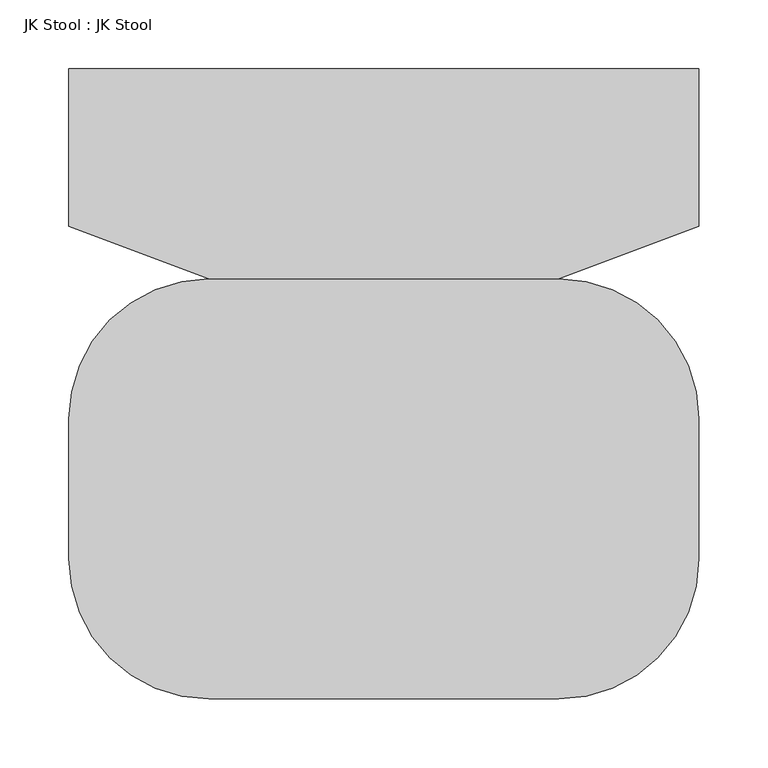
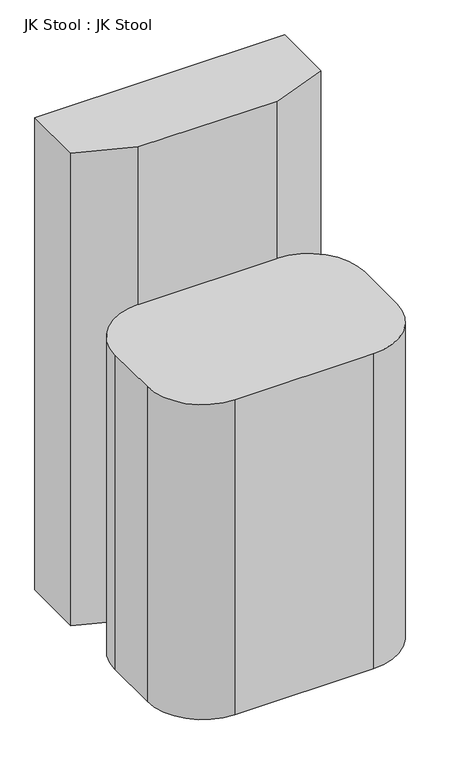
"""IFC4 building model written with IfcOpenShell, lengths in millimetres: furniture geometry, JK Stool : JK Stool."""

from ifc_helpers import new_model, si_unit, point, frame_2d, origin, origin_with_axes, place, context, project, spatial, polyline, circle_curve, trimmed, segment, composite_curve, outline, extrude, source, transform, mapped, element, save


def jk_stool_jk_stool_5b97b8dc(model_context):
    return source(origin(), model_context, "Body", "SweptSolid", [
        extrude(outline(polyline([(166.6573665, 262.1455296), (166.6573665, 147.8455296), (65.0573665, 109.7455296), (-188.9426335, 109.7455296), (-290.5426335, 147.8455296), (-290.5426335, 262.1455296), (166.6573665, 262.1455296)])), origin_with_axes(), (0.0, 0.0, 1.0), 914.4),
        extrude(outline(composite_curve([segment(trimmed(circle_curve(frame_2d((65.0573665, 8.1455296)), 101.6), [point((65.0573665, 109.7455296))], [point((166.6573665, 8.1455296))], False, "CARTESIAN"), True, "CONTINUOUS"), segment(polyline([(166.6573665, 8.1455296), (166.6573665, -93.4544704)]), True, "CONTINUOUS"), segment(trimmed(circle_curve(frame_2d((65.0573665, -93.4544704)), 101.6), [point((166.6573665, -93.4544704))], [point((65.0573665, -195.0544704))], False, "CARTESIAN"), True, "CONTINUOUS"), segment(polyline([(65.0573665, -195.0544704), (-188.9426335, -195.0544704)]), True, "CONTINUOUS"), segment(trimmed(circle_curve(frame_2d((-188.9426335, -93.4544704)), 101.6), [point((-188.9426335, -195.0544704))], [point((-290.5426335, -93.4544704))], False, "CARTESIAN"), True, "CONTINUOUS"), segment(polyline([(-290.5426335, -93.4544704), (-290.5426335, 8.1455296)]), True, "CONTINUOUS"), segment(trimmed(circle_curve(frame_2d((-188.9426335, 8.1455296)), 101.6), [point((-290.5426335, 8.1455296))], [point((-188.9426335, 109.7455296))], False, "CARTESIAN"), True, "CONTINUOUS"), segment(polyline([(-188.9426335, 109.7455296), (65.0573665, 109.7455296)]), True, "CONTINUOUS")], self_intersect=False)), origin_with_axes(), (0.0, 0.0, 1.0), 609.6),
    ])


if __name__ == "__main__":
    model = new_model("IFC4")
    model_context = context("Model", 3, world=origin())
    ifc_project = project(units=[si_unit("LENGTHUNIT", "METRE", prefix="MILLI")], contexts=[model_context])
    site = spatial("IfcSite", under=ifc_project)
    building = spatial("IfcBuilding", under=site)
    placement = place(None, origin())
    jk_stool_jk_stool_shape = jk_stool_jk_stool_5b97b8dc(model_context)
    element("IfcFurniture", 1, ObjectType="JK Stool : JK Stool", at=placement, inside=building, context=model_context, shape_type="MappedRepresentation", body=[
        mapped(jk_stool_jk_stool_shape, transform((0.0, 0.0, 0.0), x_axis=(1.0, 0.0, 0.0), y_axis=(0.0, 1.0, 0.0), z_axis=(0.0, 0.0, 1.0))),
    ])
    save(model, "model.ifc")

# Revit data of these elements
# Type "JK Stool : JK Stool"
#   Width = 1' - 6"
#   Seat Height = 2' - 0"
#   Depth = 1' - 6"
#   Corner Radius = 0' - 4"
#   Back Height = 3' - 0"
#   Arm Width = 0' - 6"
#   Status [instance default] = none
#   Default Elevation = 0
